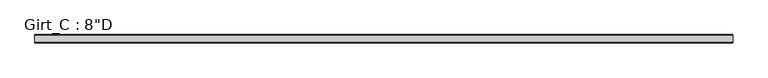
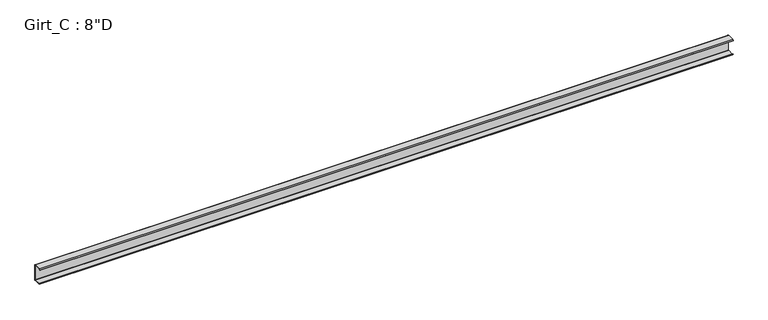
"""IFC4 building model written with IfcOpenShell, lengths in millimetres: beam geometry."""

from ifc_helpers import new_model, si_unit, point, frame, frame_2d, origin, place, context, project, spatial, polyline, circle_curve, trimmed, segment, composite_curve, outline, extrude, source, transform, mapped, element, save


def beam_405ad552(model_context):
    return source(origin(), model_context, "Body", "SweptSolid", [
        extrude(outline(composite_curve([segment(polyline([(-87.5109375, 101.6), (-3.3734375, 101.6)]), True, "CONTINUOUS"), segment(trimmed(circle_curve(frame_2d((-3.3734375, 96.8375)), 4.7625), [point((-3.3734375, 101.6))], [point((1.3890625, 96.8375))], False, "CARTESIAN"), True, "CONTINUOUS"), segment(polyline([(1.3890625, 96.8375), (1.3890625, -96.8375)]), True, "CONTINUOUS"), segment(trimmed(circle_curve(frame_2d((-3.3734375, -96.8375)), 4.7625), [point((1.3890625, -96.8375))], [point((-3.3734375, -101.6))], False, "CARTESIAN"), True, "CONTINUOUS"), segment(polyline([(-3.3734375, -101.6), (-87.5109375, -101.6), (-99.7792647, -86.979177), (-97.6510975, -85.1934327), (-86.2154765, -98.821875), (-3.2694106, -98.821875)]), True, "CONTINUOUS"), segment(trimmed(circle_curve(frame_2d((-3.3748024, -96.8389339)), 1.9857399), [point((-3.2694106, -98.821875))], [point((-1.3890625, -96.8389339))], True, "CARTESIAN"), True, "CONTINUOUS"), segment(polyline([(-1.3890625, -96.8389339), (-1.3890625, 96.8381931)]), True, "CONTINUOUS"), segment(trimmed(circle_curve(frame_2d((-3.3741066, 96.8381931)), 1.9850441), [point((-1.3890625, 96.8381931))], [point((-3.3005807, 98.821875))], True, "CARTESIAN"), True, "CONTINUOUS"), segment(polyline([(-3.3005807, 98.821875), (-86.2154765, 98.821875), (-97.6278742, 85.221109), (-99.7560415, 87.0068534), (-87.5109375, 101.6)]), True, "CONTINUOUS")], self_intersect=False)), frame((-4309.3482687, 0.0, 0.0), z_axis=(1.0, 0.0, 0.0), x_axis=(0.0, 1.0, 0.0)), (0.0, 0.0, 1.0), 8560.6732687),
    ])


if __name__ == "__main__":
    model = new_model("IFC4")
    model_context = context("Model", 3, world=origin())
    ifc_project = project(units=[si_unit("LENGTHUNIT", "METRE", prefix="MILLI")], contexts=[model_context])
    site = spatial("IfcSite", under=ifc_project)
    building = spatial("IfcBuilding", under=site)
    placement = place(None, origin())
    beam_shape = beam_405ad552(model_context)
    element("IfcBeam", 1, ObjectType="Girt_C : 8\"D", at=placement, inside=building, context=model_context, shape_type="MappedRepresentation", body=[
        mapped(beam_shape, transform((0.0, 0.0, 0.0), x_axis=(1.0, 0.0, 0.0), y_axis=(0.0, 1.0, 0.0), z_axis=(0.0, 0.0, 1.0))),
    ])
    save(model, "model.ifc")

# Revit data of these elements
# Type "Girt_C : 8\"D"
#   half leg = 0' - 1 3/4"
#   Web_Thickness = 0' - 0 7/64"
#   Length [instance default] = 10' - 0"
#   Leg_1 = 0' - 3 1/2"
#   Height = 0' - 8"
#   Structural Material [instance default] = none
# Element 1 (IfcBeam, "Girt_C : 8\"D")
#   Structural Material = GALVANIZED 'CEE' SECTION (8.0x3.5C - SEE STRUCT. DWGS)
#   Materials on its faces: "GALVANIZED 'CEE' SECTION (8.0x3.5C - SEE STRUCT. DWGS)"
# Materials
#   "GALVANIZED 'CEE' SECTION (8.0x3.5C - SEE STRUCT. DWGS)": class "Metal", colour RGB 137 146 153, transparency 0, Description = "Steel, mill finish", Cost = 0
